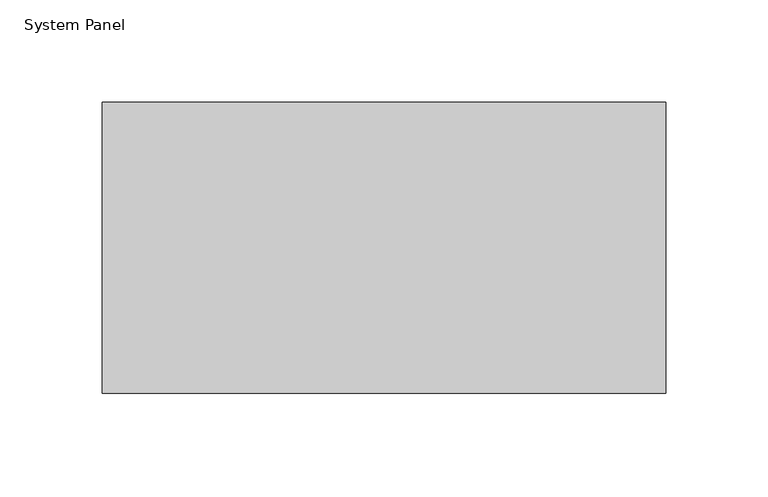
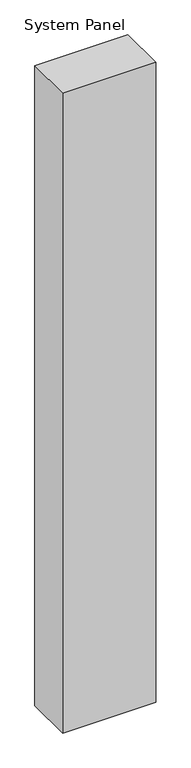
"""IFC4 building model written with IfcOpenShell, lengths in millimetres: plate geometry, System Panel : NLRS_21_CWP_hsb-vulling minerale wol 142 _gen_rsf."""

from ifc_helpers import new_model, si_unit, origin, origin_with_axes, place, context, project, spatial, polyline, outline, extrude, source, transform, mapped, element, save


def system_panel_e40bc043(model_context):
    return source(origin(), model_context, "Body", "SweptSolid", [
        extrude(outline(polyline([(137.422053, -71.0), (-137.422053, -71.0), (-137.422053, 71.0), (137.422053, 71.0), (137.422053, -71.0)])), origin_with_axes(), (0.0, 0.0, 1.0), 2000.0),
    ])


if __name__ == "__main__":
    model = new_model("IFC4")
    model_context = context("Model", 3, world=origin())
    ifc_project = project(units=[si_unit("LENGTHUNIT", "METRE", prefix="MILLI")], contexts=[model_context])
    site = spatial("IfcSite", under=ifc_project)
    building = spatial("IfcBuilding", under=site)
    placement = place(None, origin())
    system_panel_shape = system_panel_e40bc043(model_context)
    element("IfcPlate", 1, ObjectType="System Panel : NLRS_21_CWP_hsb-vulling minerale wol 142 _gen_rsf", at=placement, inside=building, context=model_context, shape_type="MappedRepresentation", body=[
        mapped(system_panel_shape, transform((0.0, 0.0, 0.0), x_axis=(1.0, 0.0, 0.0), y_axis=(0.0, 1.0, 0.0), z_axis=(0.0, 0.0, 1.0))),
    ])
    save(model, "model.ifc")

# Revit data of these elements
# Type "System Panel : NLRS_21_CWP_hsb-vulling minerale wol 142 _gen_rsf"
#   Export Type to IFC As = "IfcWall"
#   Type IfcGUID = "07M7mRoiH1CR8m_RSKIwpC"
#   Assembly Code = "21.23"
# Element 1 (IfcPlate, "System Panel : NLRS_21_CWP_hsb-vulling minerale wol 142 _gen_rsf")
#   Materials on its faces: "NLRS_m1_isolatie minerale wol_gen_rsf"
# Materials
#   "NLRS_m1_isolatie minerale wol_gen_rsf": class "M - Anorganische materialen", colour RGB 200 200 140, transparency 0, Keynote = "m1", Manufacturer = "Revit Standards Foundation", URL = "www.revitstandards.org", Description = "isolatie minerale wol", Cost = 0
